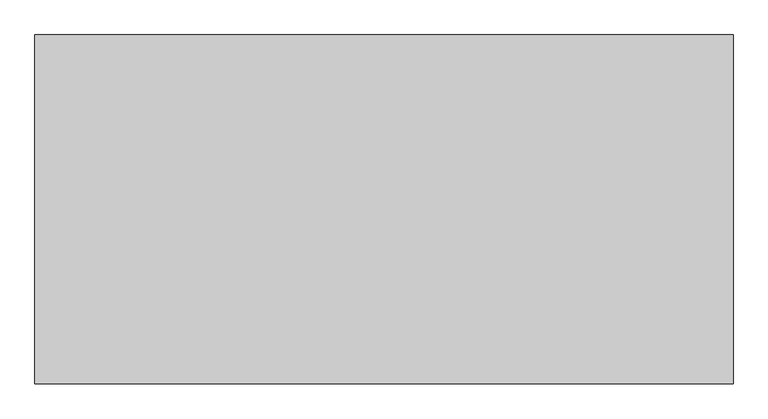
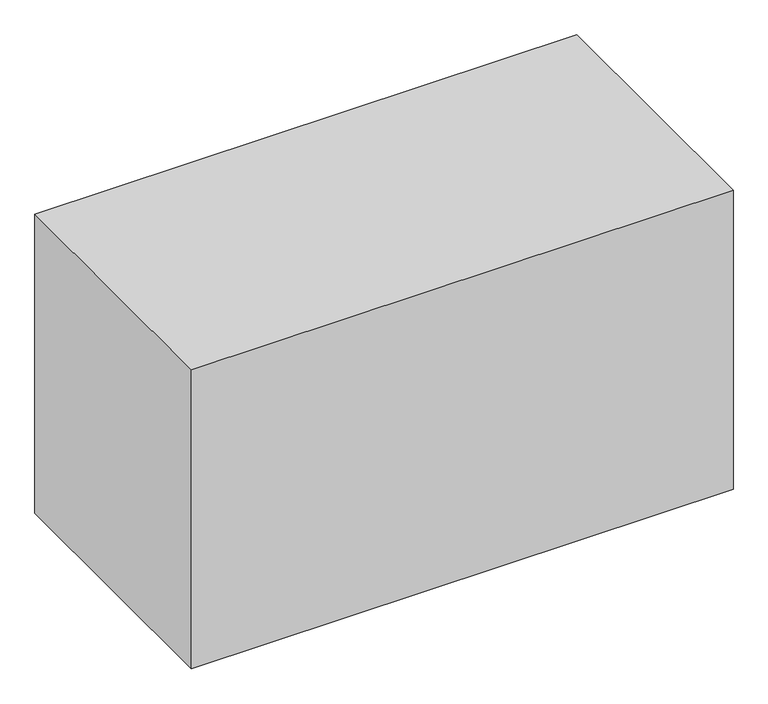
"""IFC4 building model written with IfcOpenShell, lengths in millimetres: proxy geometry, Space Planning Box_hec : Space Planning Box_hec."""

from ifc_helpers import new_model, si_unit, origin, origin_with_axes, place, context, project, spatial, polyline, outline, extrude, source, transform, mapped, element, save


def generic_models_a5818909(model_context):
    return source(origin(), model_context, "Body", "SweptSolid", [
        extrude(outline(polyline([(3000.0, 1500.0), (3000.0, -1500.0), (-3000.0, -1500.0), (-3000.0, 1500.0), (3000.0, 1500.0)])), origin_with_axes(), (0.0, 0.0, 1.0), 3500.0),
    ])


if __name__ == "__main__":
    model = new_model("IFC4")
    model_context = context("Model", 3, world=origin())
    ifc_project = project(units=[si_unit("LENGTHUNIT", "METRE", prefix="MILLI")], contexts=[model_context])
    site = spatial("IfcSite", under=ifc_project)
    building = spatial("IfcBuilding", under=site)
    placement = place(None, origin())
    generic_models_shape = generic_models_a5818909(model_context)
    element("IfcBuildingElementProxy", 1, Name="Space Planning Box_hec : Space Planning Box_hec", ObjectType="Space Planning Box_hec : Space Planning Box_hec", at=placement, inside=building, context=model_context, shape_type="MappedRepresentation", body=[
        mapped(generic_models_shape, transform((0.0, 0.0, 0.0), x_axis=(1.0, 0.0, 0.0), y_axis=(0.0, 1.0, 0.0), z_axis=(0.0, 0.0, 1.0))),
    ])
    save(model, "model.ifc")

# Revit data of these elements
# Type "Space Planning Box_hec : Space Planning Box_hec"
#   Type Comments = "..."
#   Room Name [instance default] = "?"
#   Interior Finish [instance default] = ""
#   Exterior Finish [instance default] = ""
#   Department [instance default] = ""
#   Assembly Code = "..."
#   ceiling height [instance default] = 0
#   Width [instance default] = 1524 mm
#   Program Area [instance default] = 0.00 m²
#   Length [instance default] = 1524 mm
#   Height [instance default] = 1524 mm
#   Area [instance default] = 2.32258 m²
#   Fill Color [instance default] = Cyan
#   Default Elevation = 0
# Element 1 (IfcBuildingElementProxy, "Space Planning Box_hec : Space Planning Box_hec")
#   Room Name = "Locker(M)"
#   Exterior Finish = "RF1..N/A,,EW1..N/A..N/A"
#   Department = "AR"
#   Width = 6000 mm
#   Program Area = 18.00 m²
#   Length = 3000 mm
#   Height = 3500 mm
#   Area = 18.00 m²
#   Materials on its faces: "Cyan"
# Materials
#   "Cyan": class "Generic", colour RGB 0 255 255, transparency 0.2, Cost = 0
